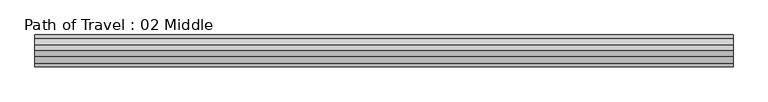
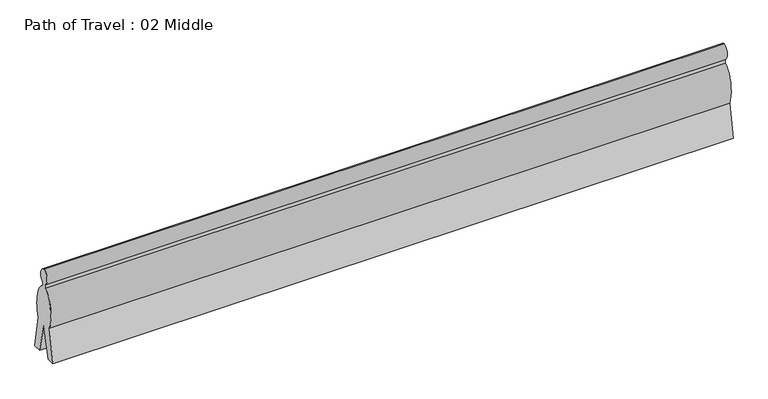
"""IFC4 building model written with IfcOpenShell, lengths in millimetres: proxy geometry, Path of Travel : 02 Middle."""

from ifc_helpers import new_model, si_unit, point, frame, origin, place, context, project, spatial, ellipse_curve, trimmed, source, transform, mapped, element, save
from ifc_brep_helpers import plane_surface, extruded_surface, advanced_brep


def path_of_travel_02_middle_d0a210c0(model_context):
    return source(origin(), model_context, "Body", "AdvancedBrep", [
        advanced_brep(
        [(227.5554837, 0.0, 1727.2), (227.5554837, 42.9018657, 1436.6534209), (227.5554837, 42.9018657, 1363.4763406), (227.5554837, 184.1186263, 643.4144547), (227.5554837, 297.5699544, 0.0), (227.5554837, 145.6574193, 0.0), (227.5554837, 0.0, 584.2), (227.5554837, -145.6574193, 0.0), (227.5554837, -297.5699544, 0.0), (227.5554837, -184.1186263, 643.4144547), (227.5554837, -42.9018657, 1363.4763406), (227.5554837, -42.9018657, 1436.6534209), (13204.6046068, 0.0, 1727.2), (13204.6046068, -42.9018657, 1436.6534209), (13204.6046068, -42.9018657, 1363.4763406), (13204.6046068, -184.1186263, 643.4144547), (13204.6046068, -297.5699544, 0.0), (13204.6046068, -145.6574193, 0.0), (13204.6046068, 0.0, 584.2), (13204.6046068, 145.6574193, 0.0), (13204.6046068, 297.5699544, 0.0), (13204.6046068, 184.1186263, 643.4144547), (13204.6046068, 42.9018657, 1363.4763406), (13204.6046068, 42.9018657, 1436.6534209)],
        [
            (0, 1, ellipse_curve(frame((227.5554837, 0.0, 1574.8), z_axis=(-1.0, 0.0, 0.0), x_axis=(0.0, 0.0, 1.0)), 152.4, 101.6)),
            (1, 2),
            (2, 3, ellipse_curve(frame((227.5554837, 0.0, 914.4), z_axis=(-1.0, 0.0, 0.0), x_axis=(0.0, 0.0, -1.0)), 457.2, 228.6)),
            (3, 4),
            (4, 5),
            (5, 6),
            (6, 7),
            (7, 8),
            (8, 9),
            (9, 10, ellipse_curve(frame((227.5554837, 0.0, 914.4), z_axis=(-1.0, 0.0, 0.0), x_axis=(0.0, 0.0, -1.0)), 457.2, 228.6)),
            (10, 11),
            (11, 0, ellipse_curve(frame((227.5554837, 0.0, 1574.8), z_axis=(-1.0, 0.0, 0.0), x_axis=(0.0, 0.0, 1.0)), 152.4, 101.6)),
            (12, 13, ellipse_curve(frame((13204.6046068, 0.0, 1574.8), z_axis=(1.0, 0.0, 0.0), x_axis=(0.0, 0.0, 1.0)), 152.4, 101.6)),
            (13, 14),
            (14, 15, ellipse_curve(frame((13204.6046068, 0.0, 914.4), z_axis=(1.0, 0.0, 0.0), x_axis=(0.0, 0.0, -1.0)), 457.2, 228.6)),
            (15, 16),
            (16, 17),
            (17, 18),
            (18, 19),
            (19, 20),
            (20, 21),
            (21, 22, ellipse_curve(frame((13204.6046068, 0.0, 914.4), z_axis=(1.0, 0.0, 0.0), x_axis=(0.0, 0.0, -1.0)), 457.2, 228.6)),
            (22, 23),
            (23, 12, ellipse_curve(frame((13204.6046068, 0.0, 1574.8), z_axis=(1.0, 0.0, 0.0), x_axis=(0.0, 0.0, 1.0)), 152.4, 101.6)),
            (0, 12),
            (23, 1),
            (22, 2),
            (21, 3),
            (20, 4),
            (19, 5),
            (18, 6),
            (17, 7),
            (16, 8),
            (15, 9),
            (14, 10),
            (13, 11),
        ],
        [
            plane_surface(frame((227.5554837, 0.0, 0.0), z_axis=(-1.0, 0.0, 0.0), x_axis=(0.0, 0.0, 1.0))),
            plane_surface(frame((13204.6046068, 0.0, 0.0), z_axis=(1.0, 0.0, 0.0), x_axis=(0.0, 0.0, 1.0))),
            extruded_surface(trimmed(ellipse_curve(frame((13204.6046068, 0.0, 1574.8), z_axis=(-1.0, 0.0, 0.0), x_axis=(0.0, 0.0, 1.0)), 152.4, 101.6), [point((13204.6046068, 0.0, 1727.2))], [point((13204.6046068, 42.9018657, 1436.6534209))], True, "CARTESIAN"), (-12977.0491231, 0.0, 0.0), 12977.0491231),
            plane_surface(frame((227.5554837, 42.9018657, 1436.6534209), z_axis=(0.0, 1.0, 0.0), x_axis=(1.0, 0.0, 0.0))),
            extruded_surface(trimmed(ellipse_curve(frame((13204.6046068, 0.0, 914.4), z_axis=(-1.0, 0.0, 0.0), x_axis=(0.0, 0.0, -1.0)), 457.2, 228.6), [point((13204.6046068, 42.9018657, 1363.4763406))], [point((13204.6046068, 184.1186263, 643.4144547))], True, "CARTESIAN"), (-12977.0491231, 0.0, 0.0), 12977.0491231),
            plane_surface(frame((227.5554837, 184.1186263, 643.4144547), z_axis=(0.0, 0.9848077530122078, 0.17364817766693205), x_axis=(1.0, 0.0, 0.0))),
            plane_surface(frame((227.5554837, 297.5699544, 0.0), z_axis=(0.0, 0.0, -1.0), x_axis=(1.0, 0.0, 0.0))),
            plane_surface(frame((227.5554837, 145.6574193, 0.0), z_axis=(0.0, -0.9702957262760199, -0.2419218955995739), x_axis=(1.0, 0.0, 0.0))),
            plane_surface(frame((227.5554837, 0.0, 584.2), z_axis=(0.0, 0.9702957262759961, -0.24192189559966923), x_axis=(1.0, 0.0, 0.0))),
            plane_surface(frame((227.5554837, -145.6574193, 0.0), z_axis=(0.0, 0.0, -1.0), x_axis=(1.0, 0.0, 0.0))),
            plane_surface(frame((227.5554837, -297.5699544, 0.0), z_axis=(0.0, -0.984807753012208, 0.17364817766693066), x_axis=(1.0, 0.0, 0.0))),
            extruded_surface(trimmed(ellipse_curve(frame((13204.6046068, 0.0, 914.4), z_axis=(-1.0, 0.0, 0.0), x_axis=(0.0, 0.0, -1.0)), 457.2, 228.6), [point((13204.6046068, -184.1186263, 643.4144547))], [point((13204.6046068, -42.9018657, 1363.4763406))], True, "CARTESIAN"), (-12977.0491231, 0.0, 0.0), 12977.0491231),
            plane_surface(frame((227.5554837, -42.9018657, 1363.4763406), z_axis=(0.0, -1.0, 0.0), x_axis=(1.0, 0.0, 0.0))),
            extruded_surface(trimmed(ellipse_curve(frame((13204.6046068, 0.0, 1574.8), z_axis=(-1.0, 0.0, 0.0), x_axis=(0.0, 0.0, 1.0)), 152.4, 101.6), [point((13204.6046068, -42.9018657, 1436.6534209))], [point((13204.6046068, 0.0, 1727.2))], True, "CARTESIAN"), (-12977.0491231, 0.0, 0.0), 12977.0491231),
        ],
        [
            (0, [[1, 2, 3, 4, 5, 6, 7, 8, 9, 10, 11, 12]]),
            (1, [[13, 14, 15, 16, 17, 18, 19, 20, 21, 22, 23, 24]]),
            (2, [[-1, 25, -24, 26]]),
            (3, [[-2, -26, -23, 27]]),
            (4, [[-3, -27, -22, 28]]),
            (5, [[-4, -28, -21, 29]]),
            (6, [[-5, -29, -20, 30]]),
            (7, [[-6, -30, -19, 31]]),
            (8, [[-7, -31, -18, 32]]),
            (9, [[-8, -32, -17, 33]]),
            (10, [[-9, -33, -16, 34]]),
            (11, [[-10, -34, -15, 35]]),
            (12, [[-11, -35, -14, 36]]),
            (13, [[-12, -36, -13, -25]]),
        ],
    ),
    ])


if __name__ == "__main__":
    model = new_model("IFC4")
    model_context = context("Model", 3, world=origin())
    ifc_project = project(units=[si_unit("LENGTHUNIT", "METRE", prefix="MILLI")], contexts=[model_context])
    site = spatial("IfcSite", under=ifc_project)
    building = spatial("IfcBuilding", under=site)
    placement = place(None, origin())
    path_of_travel_02_middle_shape = path_of_travel_02_middle_d0a210c0(model_context)
    element("IfcBuildingElementProxy", 1, Name="Path of Travel : 02 Middle", ObjectType="Path of Travel : 02 Middle", at=placement, inside=building, context=model_context, shape_type="MappedRepresentation", body=[
        mapped(path_of_travel_02_middle_shape, transform((0.0, 0.0, 0.0), x_axis=(1.0, 0.0, 0.0), y_axis=(0.0, 1.0, 0.0), z_axis=(0.0, 0.0, 1.0))),
    ])
    save(model, "model.ifc")

# Revit data of these elements
# Type "Path of Travel : 02 Middle"
#   Path of Egress [instance default] = 4' - 0"
#   built-in parameter 1001306 [instance default] = 4 (stored number, unit not read)
#   Dot at Start = no
#   Arrow in Middle = yes
#   Arrow at End = no
#   Egress Path = none
# Element 1 (IfcBuildingElementProxy, "Path of Travel : 02 Middle")
#   Path of Egress = 42' - 6.90745"
#   built-in parameter 1001306 = 42.5756 (stored number, unit not read)
#   Materials on its faces: "Egress Path Solid"
# Materials
#   "Egress Path Solid": class "Unassigned", colour RGB 255 128 64, transparency 0.75, Comments = "Rendering appearance not upgraded "
